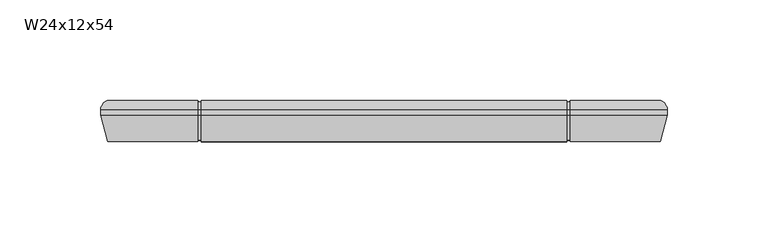
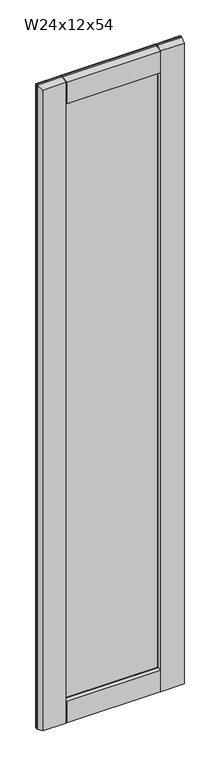
"""IFC4 building model written with IfcOpenShell, lengths in millimetres: furniture geometry, Cabinet-Wall-Merillat-Double_Door-Marlin : W24x12x54."""

from ifc_helpers import new_model, si_unit, frame, origin, place, context, project, spatial, polyline, circle_curve, ellipse_curve, outline, extrude, source, transform, mapped, element, save
from ifc_brep_helpers import plane_surface, cylinder_surface, advanced_brep


def w24x12x54_cfe01b16(model_context):
    return source(origin(), model_context, "Body", "SolidModel", [
        advanced_brep(
        [(541.0528392, 382.5621, 2108.2), (541.0528392, 382.5621, 787.4), (537.9563467, 387.0325, 790.4964925), (537.9563467, 387.0325, 2105.1035075), (541.0528392, 379.7935, 2108.2), (541.0528392, 379.7935, 787.4), (537.5476392, 366.7125, 2104.6948), (537.5476392, 366.7125, 790.9052), (492.8516765, 366.7125, 2059.9988372), (492.4815448, 367.50625, 2059.6287055), (490.4003857, 371.96931, 2057.5475465), (490.4003857, 371.96931, 838.0524535), (492.4815448, 367.50625, 835.9712945), (492.8516765, 366.7125, 835.6011628), (491.8001552, 374.2094093, 2058.947316), (491.8001552, 374.2094093, 836.652684), (506.1278392, 374.4595, 2073.275), (506.1278392, 374.4595, 822.325), (506.1278392, 379.2855, 2073.275), (506.1278392, 379.2855, 822.325), (491.8001552, 379.5355907, 2058.947316), (491.8001552, 379.5355907, 836.652684), (490.4003857, 381.77569, 2057.5475465), (490.4003857, 381.77569, 838.0524535), (492.4815448, 386.23875, 2059.6287055), (492.848809, 387.0263508, 2059.9959698), (492.8516765, 387.0325, 835.6011628), (492.4815448, 386.23875, 835.9712945), (263.1618317, 387.0325, 790.4964925), (308.2295579, 387.0325, 790.4964925), (308.2295579, 382.5621, 787.4), (260.0653392, 382.5621, 787.4), (492.848809, 382.5621, 787.4), (492.848809, 387.0325, 790.4964925), (491.261309, 382.5621, 787.4), (309.8170579, 382.5621, 787.4), (309.8170579, 387.0325, 790.4964925), (491.261309, 387.0325, 790.4964925), (308.2295579, 379.7935, 787.4), (260.0653392, 379.7935, 787.4), (492.848809, 379.7935, 787.4), (491.261309, 379.7935, 787.4), (309.8170579, 379.7935, 787.4), (308.2295579, 366.7125, 790.9052), (263.5705392, 366.7125, 790.9052), (491.261309, 366.7125, 790.9052), (309.8170579, 366.7125, 790.9052), (492.848809, 366.7125, 790.9052), (310.7177927, 371.96931, 838.0524535), (308.6366337, 367.50625, 835.9712945), (309.8170579, 367.50625, 835.9712945), (309.8170579, 366.7125, 835.6011628), (491.261309, 366.7125, 835.6011628), (491.261309, 367.50625, 835.9712945), (309.3180233, 374.2094093, 836.652684), (294.9903392, 374.4595, 822.325), (294.9903392, 379.2855, 822.325), (309.3180233, 379.5355907, 836.652684), (310.7177927, 381.77569, 838.0524535), (491.261309, 386.23875, 835.9712945), (491.261309, 387.0325, 835.6011628), (309.8170579, 387.0325, 835.6011628), (309.8170579, 386.23875, 835.9712945), (308.6366337, 386.23875, 835.9712945), (260.0653392, 382.5621, 2108.2), (263.1618317, 387.0325, 2105.1035075), (260.0653392, 379.7935, 2108.2), (263.5705392, 366.7125, 2104.6948), (308.266502, 366.7125, 835.6011628), (310.7177927, 371.96931, 2057.5475465), (308.6366337, 367.50625, 2059.6287055), (308.266502, 366.7125, 2059.9988372), (309.3180233, 374.2094093, 2058.947316), (294.9903392, 374.4595, 2073.275), (294.9903392, 379.2855, 2073.275), (309.3180233, 379.5355907, 2058.947316), (310.7177927, 381.77569, 2057.5475465), (308.266502, 387.0325, 835.6011628), (308.266502, 387.0325, 2059.9988372), (308.6366337, 386.23875, 2059.6287055), (492.848809, 387.0325, 2105.1035075), (492.848809, 382.5621, 2108.2), (308.2295579, 382.5621, 2108.2), (308.2295579, 387.0325, 2105.1035075), (309.8170579, 382.5621, 2108.2), (491.261309, 382.5621, 2108.2), (491.261309, 387.0325, 2105.1035075), (309.8170579, 387.0325, 2105.1035075), (492.848809, 379.7935, 2108.2), (308.2295579, 379.7935, 2108.2), (309.8170579, 379.7935, 2108.2), (491.261309, 379.7935, 2108.2), (492.848809, 366.7125, 2104.6948), (308.2295579, 366.7125, 2104.6948), (309.8170579, 366.7125, 2104.6948), (491.261309, 366.7125, 2104.6948), (309.8170579, 366.7125, 2059.9988372), (491.261309, 366.7125, 2059.9988372), (491.261309, 367.50625, 2059.6287055), (309.8170579, 367.50625, 2059.6287055), (309.8170579, 386.23875, 2059.6287055), (309.8170579, 387.0325, 2059.9988372), (491.261309, 387.0325, 2059.9988372), (491.261309, 386.23875, 2059.6287055), (309.8170579, 386.23875, 2104.9526052), (309.8170579, 382.5621, 2107.40625), (309.8170579, 379.8980037, 2107.40625), (309.8170579, 367.50625, 2104.0857412), (308.2295579, 367.50625, 2059.6287055), (308.2295579, 367.50625, 2104.0857412), (308.2295579, 379.8980037, 2107.40625), (308.2295579, 382.5621, 2107.40625), (308.2295579, 386.23875, 2104.9526052), (308.2295579, 386.23875, 2059.6287055), (492.848809, 386.23875, 2059.6287055), (492.848809, 386.23875, 2104.9526052), (492.848809, 382.5621, 2107.40625), (492.848809, 379.8980037, 2107.40625), (492.848809, 367.50625, 2104.0857412), (492.848809, 367.50625, 2059.6287055), (491.261309, 367.50625, 2104.0857412), (491.261309, 379.8980037, 2107.40625), (491.261309, 382.5621, 2107.40625), (491.261309, 386.23875, 2104.9526052), (492.848809, 367.50625, 835.9712945), (492.848809, 367.50625, 791.5142588), (492.848809, 379.8980037, 788.19375), (492.848809, 382.5621, 788.19375), (492.848809, 386.23875, 790.6473948), (492.848809, 386.23875, 835.9712945), (491.261309, 386.23875, 790.6473948), (491.261309, 382.5621, 788.19375), (491.261309, 379.8980037, 788.19375), (491.261309, 367.50625, 791.5142588), (309.8170579, 367.50625, 791.5142588), (309.8170579, 379.8980037, 788.19375), (309.8170579, 382.5621, 788.19375), (309.8170579, 386.23875, 790.6473948), (308.2295579, 386.23875, 835.9712945), (308.2295579, 386.23875, 790.6473948), (308.2295579, 382.5621, 788.19375), (308.2295579, 379.8980037, 788.19375), (308.2295579, 367.50625, 791.5142588), (308.2295579, 367.50625, 835.9712945)],
        [
            (0, 1),
            (1, 2, ellipse_curve(frame((536.2776392, 382.5621, 792.1752), z_axis=(0.7071067811865475, 0.0, 0.7071067811865475), x_axis=(-0.7071067811865474, 0.0, 0.7071067811865476)), 6.7531526, 4.7752)),
            (2, 3),
            (3, 0, ellipse_curve(frame((536.2776392, 382.5621, 2103.4248), z_axis=(0.7071067811865475, 0.0, -0.7071067811865475), x_axis=(0.7071067811865474, 0.0, 0.7071067811865476)), 6.7531526, 4.7752)),
            (0, 4),
            (4, 5),
            (5, 1),
            (4, 6),
            (6, 7),
            (7, 5),
            (8, 9),
            (9, 10),
            (10, 11),
            (11, 12),
            (12, 13),
            (13, 8),
            (10, 14, ellipse_curve(frame((491.8276392, 372.6348492, 2058.9748), z_axis=(0.7071067811865475, 0.0, -0.7071067811865475), x_axis=(0.7071067811865474, 0.0, 0.7071067811865476)), 2.2271035, 1.5748)),
            (14, 15),
            (15, 11, ellipse_curve(frame((491.8276392, 372.6348492, 836.6252), z_axis=(0.7071067811865475, 0.0, 0.7071067811865475), x_axis=(-0.7071067811865474, 0.0, 0.7071067811865476)), 2.2271035, 1.5748)),
            (14, 16),
            (16, 17),
            (17, 15),
            (16, 18),
            (18, 19),
            (19, 17),
            (18, 20),
            (20, 21),
            (21, 19),
            (20, 22, ellipse_curve(frame((491.8276392, 381.1101508, 2058.9748), z_axis=(0.7071067811865475, 0.0, -0.7071067811865475), x_axis=(0.7071067811865474, 0.0, 0.7071067811865476)), 2.2271035, 1.5748)),
            (22, 23),
            (23, 21, ellipse_curve(frame((491.8276392, 381.1101508, 836.6252), z_axis=(0.7071067811865475, 0.0, 0.7071067811865475), x_axis=(-0.7071067811865474, 0.0, 0.7071067811865476)), 2.2271035, 1.5748)),
            (22, 24),
            (24, 25),
            (25, 26),
            (26, 27),
            (27, 23),
            (28, 29),
            (29, 30, circle_curve(frame((308.2295579, 382.5621, 792.1752), z_axis=(-1.0, 0.0, 0.0), x_axis=(0.0, -1.0, 0.0)), 4.7752)),
            (30, 31),
            (31, 28, ellipse_curve(frame((264.8405392, 382.5621, 792.1752), z_axis=(0.7071067811865475, 0.0, -0.7071067811865475), x_axis=(0.7071067811865476, 0.0, 0.7071067811865474)), 6.7531526, 4.7752)),
            (1, 32),
            (32, 33, circle_curve(frame((492.848809, 382.5621, 792.1752), z_axis=(1.0, 0.0, 0.0), x_axis=(0.0, -1.0, 0.0)), 4.7752)),
            (33, 2),
            (34, 35),
            (35, 36, circle_curve(frame((309.8170579, 382.5621, 792.1752), z_axis=(1.0, 0.0, 0.0), x_axis=(0.0, -1.0, 0.0)), 4.7752)),
            (36, 37),
            (37, 34, circle_curve(frame((491.261309, 382.5621, 792.1752), z_axis=(-1.0, 0.0, 0.0), x_axis=(0.0, -1.0, 0.0)), 4.7752)),
            (30, 38),
            (38, 39),
            (39, 31),
            (5, 40),
            (40, 32),
            (41, 42),
            (42, 35),
            (34, 41),
            (38, 43),
            (43, 44),
            (44, 39),
            (45, 46),
            (46, 42),
            (41, 45),
            (7, 47),
            (47, 40),
            (48, 49),
            (49, 50),
            (50, 51),
            (51, 52),
            (52, 53),
            (53, 12),
            (11, 48),
            (15, 54),
            (54, 48, ellipse_curve(frame((309.2905392, 372.6348492, 836.6252), z_axis=(0.7071067811865475, 0.0, -0.7071067811865475), x_axis=(0.7071067811865476, 0.0, 0.7071067811865474)), 2.2271035, 1.5748)),
            (17, 55),
            (55, 54),
            (19, 56),
            (56, 55),
            (21, 57),
            (57, 56),
            (23, 58),
            (58, 57, ellipse_curve(frame((309.2905392, 381.1101508, 836.6252), z_axis=(0.7071067811865475, 0.0, -0.7071067811865475), x_axis=(0.7071067811865476, 0.0, 0.7071067811865474)), 2.2271035, 1.5748)),
            (27, 59),
            (59, 60),
            (60, 61),
            (61, 62),
            (62, 63),
            (63, 58),
            (31, 64),
            (64, 65, ellipse_curve(frame((264.8405392, 382.5621, 2103.4248), z_axis=(-0.7071067811865475, 0.0, -0.7071067811865475), x_axis=(0.7071067811865474, 0.0, -0.7071067811865476)), 6.7531526, 4.7752)),
            (65, 28),
            (39, 66),
            (66, 64),
            (44, 67),
            (67, 66),
            (68, 49),
            (48, 69),
            (69, 70),
            (70, 71),
            (71, 68),
            (54, 72),
            (72, 69, ellipse_curve(frame((309.2905392, 372.6348492, 2058.9748), z_axis=(-0.7071067811865475, 0.0, -0.7071067811865475), x_axis=(0.7071067811865474, 0.0, -0.7071067811865476)), 2.2271035, 1.5748)),
            (55, 73),
            (73, 72),
            (56, 74),
            (74, 73),
            (57, 75),
            (75, 74),
            (58, 76),
            (76, 75, ellipse_curve(frame((309.2905392, 381.1101508, 2058.9748), z_axis=(-0.7071067811865475, 0.0, -0.7071067811865475), x_axis=(0.7071067811865474, 0.0, -0.7071067811865476)), 2.2271035, 1.5748)),
            (63, 77),
            (77, 78),
            (78, 79),
            (79, 76),
            (3, 80),
            (80, 81, circle_curve(frame((492.848809, 382.5621, 2103.4248), z_axis=(1.0, 0.0, 0.0), x_axis=(0.0, -1.0, 0.0)), 4.7752)),
            (81, 0),
            (64, 82),
            (82, 83, circle_curve(frame((308.2295579, 382.5621, 2103.4248), z_axis=(-1.0, 0.0, 0.0), x_axis=(0.0, -1.0, 0.0)), 4.7752)),
            (83, 65),
            (84, 85),
            (85, 86, circle_curve(frame((491.261309, 382.5621, 2103.4248), z_axis=(-1.0, 0.0, 0.0), x_axis=(0.0, -1.0, 0.0)), 4.7752)),
            (86, 87),
            (87, 84, circle_curve(frame((309.8170579, 382.5621, 2103.4248), z_axis=(1.0, 0.0, 0.0), x_axis=(0.0, -1.0, 0.0)), 4.7752)),
            (81, 88),
            (88, 4),
            (66, 89),
            (89, 82),
            (90, 91),
            (91, 85),
            (84, 90),
            (88, 92),
            (92, 6),
            (67, 93),
            (93, 89),
            (94, 95),
            (95, 91),
            (90, 94),
            (51, 46),
            (45, 52),
            (43, 68),
            (71, 93),
            (92, 8),
            (13, 47),
            (96, 97),
            (97, 95),
            (94, 96),
            (9, 98),
            (98, 97),
            (96, 99),
            (99, 70),
            (69, 10),
            (72, 14),
            (73, 16),
            (74, 18),
            (75, 20),
            (76, 22),
            (79, 100),
            (100, 101),
            (101, 102),
            (102, 103),
            (103, 24),
            (33, 26),
            (25, 80),
            (36, 61),
            (60, 37),
            (83, 78),
            (77, 29),
            (86, 102),
            (101, 87),
            (100, 104),
            (104, 105, circle_curve(frame((309.8170579, 382.5621, 2103.4248), z_axis=(1.0, 0.0, 0.0), x_axis=(0.0, 0.0, 1.0)), 3.98145)),
            (105, 106),
            (106, 107),
            (107, 99),
            (71, 108),
            (108, 109),
            (109, 110),
            (110, 111),
            (111, 112, circle_curve(frame((308.2295579, 382.5621, 2103.4248), z_axis=(-1.0, 0.0, 0.0), x_axis=(0.0, 0.0, 1.0)), 3.98145)),
            (112, 113),
            (113, 78),
            (113, 79),
            (112, 104),
            (111, 105),
            (110, 106),
            (109, 107),
            (108, 70),
            (25, 114),
            (114, 115),
            (115, 116, circle_curve(frame((492.848809, 382.5621, 2103.4248), z_axis=(1.0, 0.0, 0.0), x_axis=(0.0, 0.0, 1.0)), 3.98145)),
            (116, 117),
            (117, 118),
            (118, 119),
            (119, 8),
            (98, 120),
            (120, 121),
            (121, 122),
            (122, 123, circle_curve(frame((491.261309, 382.5621, 2103.4248), z_axis=(-1.0, 0.0, 0.0), x_axis=(0.0, 0.0, 1.0)), 3.98145)),
            (123, 103),
            (24, 114),
            (123, 115),
            (122, 116),
            (121, 117),
            (120, 118),
            (9, 119),
            (13, 124),
            (124, 125),
            (125, 126),
            (126, 127),
            (127, 128, circle_curve(frame((492.848809, 382.5621, 792.1752), z_axis=(1.0, 0.0, 0.0), x_axis=(0.0, 0.0, 1.0)), 3.98145)),
            (128, 129),
            (129, 26),
            (59, 130),
            (130, 131, circle_curve(frame((491.261309, 382.5621, 792.1752), z_axis=(-1.0, 0.0, 0.0), x_axis=(0.0, 0.0, 1.0)), 3.98145)),
            (131, 132),
            (132, 133),
            (133, 53),
            (12, 124),
            (133, 125),
            (132, 126),
            (131, 127),
            (130, 128),
            (27, 129),
            (50, 134),
            (134, 135),
            (135, 136),
            (136, 137, circle_curve(frame((309.8170579, 382.5621, 792.1752), z_axis=(1.0, 0.0, 0.0), x_axis=(0.0, 0.0, 1.0)), 3.98145)),
            (137, 62),
            (138, 139),
            (139, 140, circle_curve(frame((308.2295579, 382.5621, 792.1752), z_axis=(-1.0, 0.0, 0.0), x_axis=(0.0, 0.0, 1.0)), 3.98145)),
            (140, 141),
            (141, 142),
            (142, 143),
            (143, 68),
            (77, 138),
            (63, 138),
            (143, 49),
            (142, 134),
            (141, 135),
            (140, 136),
            (139, 137),
        ],
        [
            cylinder_surface(frame((536.2776392, 382.5621, 2108.2), z_axis=(0.0, 0.0, 1.0), x_axis=(0.0, -1.0, 0.0)), 4.7752),
            plane_surface(frame((541.0528392, 382.5621, 2108.2), z_axis=(1.0, 0.0, 0.0), x_axis=(0.0, 0.0, -1.0))),
            plane_surface(frame((541.0528392, 379.7935, 2108.2), z_axis=(0.9659229350723619, -0.25882983502910506, 0.0), x_axis=(0.0, 0.0, -1.0))),
            plane_surface(frame((492.8516765, 366.7125, 2059.9988372), z_axis=(-0.9063077870366099, -0.4226182617407856, 0.0), x_axis=(0.0, 0.0, -1.0))),
            cylinder_surface(frame((491.8276392, 372.6348492, 2108.2), z_axis=(0.0, 0.0, 1.0000000000000002), x_axis=(-0.01745240643729364, 0.9998476951563912, 0.0)), 1.5748),
            plane_surface(frame((491.8001552, 374.2094093, 2058.947316), z_axis=(-0.017452406437322144, 0.9998476951563906, 0.0), x_axis=(0.0, 0.0, -1.0))),
            plane_surface(frame((506.1278392, 374.4595, 2073.275), z_axis=(-1.0, 0.0, 0.0), x_axis=(0.0, 0.0, -1.0))),
            plane_surface(frame((506.1278392, 379.2855, 2073.275), z_axis=(-0.01745240643727848, -0.9998476951563914, 0.0), x_axis=(0.0, 0.0, -1.0))),
            cylinder_surface(frame((491.8276392, 381.1101508, 2108.2), z_axis=(0.0, 0.0, 1.0000000000000002), x_axis=(-0.9063077870367326, 0.42261826174052236, 0.0)), 1.5748),
            plane_surface(frame((490.4003857, 381.77569, 2057.5475465), z_axis=(-0.9063077870366333, 0.4226182617407352, 0.0), x_axis=(0.0, 0.0, -1.0))),
            cylinder_surface(frame((541.0528392, 382.5621, 792.1752), z_axis=(1.0, 0.0, 0.0), x_axis=(0.0, -1.0, 0.0)), 4.7752),
            plane_surface(frame((541.0528392, 382.5621, 787.4), z_axis=(0.0, 0.0, -1.0), x_axis=(-1.0, 0.0, 0.0))),
            plane_surface(frame((541.0528392, 379.7935, 787.4), z_axis=(0.0, -0.2588298350291095, -0.9659229350723607), x_axis=(-1.0, 0.0, 0.0))),
            plane_surface(frame((492.8516765, 366.7125, 835.6011628), z_axis=(0.0, -0.42261826174078143, 0.9063077870366119), x_axis=(-1.0, 0.0, 0.0))),
            cylinder_surface(frame((541.0528392, 372.6348492, 836.6252), z_axis=(1.0000000000000002, 0.0, 0.0), x_axis=(0.0, 0.9998476951563913, 0.017452406437289025)), 1.5748),
            plane_surface(frame((491.8001552, 374.2094093, 836.652684), z_axis=(0.0, 0.9998476951563907, 0.01745240643731753), x_axis=(-1.0, 0.0, 0.0))),
            plane_surface(frame((506.1278392, 374.4595, 822.325), z_axis=(0.0, 0.0, 1.0), x_axis=(-1.0, 0.0, 0.0))),
            plane_surface(frame((506.1278392, 379.2855, 822.325), z_axis=(0.0, -0.9998476951563913, 0.017452406437283095), x_axis=(-1.0, 0.0, 0.0))),
            cylinder_surface(frame((541.0528392, 381.1101508, 836.6252), z_axis=(1.0000000000000002, 0.0, 0.0), x_axis=(0.0, 0.4226182617405265, 0.9063077870367306)), 1.5748),
            plane_surface(frame((490.4003857, 381.77569, 838.0524535), z_axis=(0.0, 0.4226182617407394, 0.9063077870366314), x_axis=(-1.0, 0.0, 0.0))),
            cylinder_surface(frame((264.8405392, 382.5621, 787.4), z_axis=(0.0, 0.0, -1.0), x_axis=(0.0, -1.0, 0.0)), 4.7752),
            plane_surface(frame((260.0653392, 382.5621, 787.4), z_axis=(-1.0, 0.0, 0.0), x_axis=(0.0, 0.0, 1.0))),
            plane_surface(frame((260.0653392, 379.7935, 787.4), z_axis=(-0.9659229350723619, -0.25882983502910506, 0.0), x_axis=(0.0, 0.0, 1.0))),
            plane_surface(frame((308.266502, 366.7125, 835.6011628), z_axis=(0.9063077870366099, -0.4226182617407856, 0.0), x_axis=(0.0, 0.0, 1.0))),
            cylinder_surface(frame((309.2905392, 372.6348492, 787.4), z_axis=(0.0, 0.0, -1.0000000000000002), x_axis=(0.01745240643729364, 0.9998476951563912, 0.0)), 1.5748),
            plane_surface(frame((309.3180233, 374.2094093, 836.652684), z_axis=(0.017452406437322144, 0.9998476951563906, 0.0), x_axis=(0.0, 0.0, 1.0))),
            plane_surface(frame((294.9903392, 374.4595, 822.325), z_axis=(1.0, 0.0, 0.0), x_axis=(0.0, 0.0, 1.0))),
            plane_surface(frame((294.9903392, 379.2855, 822.325), z_axis=(0.01745240643727848, -0.9998476951563914, 0.0), x_axis=(0.0, 0.0, 1.0))),
            cylinder_surface(frame((309.2905392, 381.1101508, 787.4), z_axis=(0.0, 0.0, -1.0000000000000002), x_axis=(0.9063077870367326, 0.42261826174052236, 0.0)), 1.5748),
            plane_surface(frame((310.7177927, 381.77569, 838.0524535), z_axis=(0.9063077870366333, 0.4226182617407352, 0.0), x_axis=(0.0, 0.0, 1.0))),
            cylinder_surface(frame((260.0653392, 382.5621, 2103.4248), z_axis=(-1.0, 0.0, 0.0), x_axis=(0.0, -1.0, 0.0)), 4.7752),
            plane_surface(frame((260.0653392, 382.5621, 2108.2), z_axis=(0.0, 0.0, 1.0), x_axis=(1.0, 0.0, 0.0))),
            plane_surface(frame((260.0653392, 379.7935, 2108.2), z_axis=(0.0, -0.2588298350291006, 0.9659229350723632), x_axis=(1.0, 0.0, 0.0))),
            plane_surface(frame((263.5705392, 366.7125, 2104.6948), z_axis=(0.0, -1.0, 0.0), x_axis=(1.0, 0.0, 0.0))),
            plane_surface(frame((308.266502, 366.7125, 2059.9988372), z_axis=(0.0, -0.42261826174078976, -0.9063077870366079), x_axis=(1.0, 0.0, 0.0))),
            cylinder_surface(frame((260.0653392, 372.6348492, 2058.9748), z_axis=(-1.0000000000000002, 0.0, 0.0), x_axis=(0.0, 0.999847695156391, -0.017452406437298253)), 1.5748),
            plane_surface(frame((309.3180233, 374.2094093, 2058.947316), z_axis=(0.0, 0.9998476951563905, -0.01745240643732676), x_axis=(1.0, 0.0, 0.0))),
            plane_surface(frame((294.9903392, 374.4595, 2073.275), z_axis=(0.0, 0.0, -1.0), x_axis=(1.0, 0.0, 0.0))),
            plane_surface(frame((294.9903392, 379.2855, 2073.275), z_axis=(0.0, -0.9998476951563915, -0.017452406437273867), x_axis=(1.0, 0.0, 0.0))),
            cylinder_surface(frame((260.0653392, 381.1101508, 2058.9748), z_axis=(-1.0000000000000002, 0.0, 0.0), x_axis=(0.0, 0.4226182617405182, -0.9063077870367346)), 1.5748),
            plane_surface(frame((310.7177927, 381.77569, 2057.5475465), z_axis=(0.0, 0.422618261740731, -0.9063077870366353), x_axis=(1.0, 0.0, 0.0))),
            plane_surface(frame((308.266502, 387.0325, 2059.9988372), z_axis=(0.0, 1.0, 0.0), x_axis=(1.0, 0.0, 0.0))),
            plane_surface(frame((309.8170579, 387.0325, 2059.9988372), z_axis=(-1.0000000000000002, 0.0, 0.0), x_axis=(0.0, -0.9063077870366177, -0.4226182617407689))),
            plane_surface(frame((308.2295579, 387.0325, 2059.9988372), z_axis=(1.0000000000000002, 0.0, 0.0), x_axis=(0.0, 0.9063077870366177, 0.4226182617407689))),
            plane_surface(frame((309.8170579, 387.0325, 2059.9988372), z_axis=(0.0, -0.4226182617407689, 0.9063077870366177), x_axis=(-1.0, 0.0, 0.0))),
            plane_surface(frame((309.8170579, 386.23875, 2059.6287055), z_axis=(0.0, 1.0, 0.0), x_axis=(-1.0, 0.0, 0.0))),
            cylinder_surface(frame((308.2295579, 382.5621, 2103.4248), z_axis=(-1.0, 0.0, 0.0), x_axis=(0.0, 0.0, 1.0)), 3.98145),
            plane_surface(frame((309.8170579, 382.5621, 2107.40625), z_axis=(0.0, 0.0, 1.0), x_axis=(-1.0, 0.0, 0.0))),
            plane_surface(frame((309.8170579, 379.8980037, 2107.40625), z_axis=(0.0, -0.2588298350291571, 0.965922935072348), x_axis=(-1.0, 0.0, 0.0))),
            plane_surface(frame((309.8170579, 367.50625, 2104.0857412), z_axis=(0.0, -1.0, 0.0), x_axis=(-1.0, 0.0, 0.0))),
            plane_surface(frame((309.8170579, 367.50625, 2059.6287055), z_axis=(0.0, 0.4226182617408151, 0.906307787036596), x_axis=(-1.0, 0.0, 0.0))),
            plane_surface(frame((492.848809, 387.0325, 2059.9988372), z_axis=(-1.0, 0.0, 0.0), x_axis=(0.0, -0.9063077870366254, -0.42261826174075223))),
            plane_surface(frame((491.261309, 387.0325, 2059.9988372), z_axis=(1.0, 0.0, 0.0), x_axis=(0.0, 0.9063077870366254, 0.42261826174075223))),
            plane_surface(frame((492.848809, 387.0325, 2059.9988372), z_axis=(0.0, -0.42261826174075223, 0.9063077870366254), x_axis=(-1.0, 0.0, 0.0))),
            plane_surface(frame((492.848809, 386.23875, 2059.6287055), z_axis=(0.0, 1.0, 0.0), x_axis=(-1.0, 0.0, 0.0))),
            cylinder_surface(frame((491.261309, 382.5621, 2103.4248), z_axis=(-1.0, 0.0, 0.0), x_axis=(0.0, 0.0, 1.0)), 3.98145),
            plane_surface(frame((492.848809, 382.5621, 2107.40625), z_axis=(0.0, 0.0, 1.0), x_axis=(-1.0, 0.0, 0.0))),
            plane_surface(frame((492.848809, 379.8980037, 2107.40625), z_axis=(0.0, -0.258829835029159, 0.9659229350723475), x_axis=(-1.0, 0.0, 0.0))),
            plane_surface(frame((492.848809, 367.50625, 2104.0857412), z_axis=(0.0, -1.0, 0.0), x_axis=(-1.0, 0.0, 0.0))),
            plane_surface(frame((492.848809, 367.50625, 2059.6287055), z_axis=(0.0, 0.4226182617408322, 0.9063077870365881), x_axis=(-1.0, 0.0, 0.0))),
            plane_surface(frame((492.848809, 382.5621, 796.9504), z_axis=(-1.0, 0.0, 0.0), x_axis=(0.0, 1.0, 0.0))),
            plane_surface(frame((491.261309, 382.5621, 796.9504), z_axis=(1.0, 0.0, 0.0), x_axis=(0.0, -1.0, 0.0))),
            plane_surface(frame((492.848809, 366.7125, 835.6011628), z_axis=(0.0, 0.4226182617407559, -0.9063077870366237), x_axis=(-1.0, 0.0, 0.0))),
            plane_surface(frame((492.848809, 367.50625, 835.9712945), z_axis=(0.0, -1.0, 0.0), x_axis=(-1.0, 0.0, 0.0))),
            plane_surface(frame((492.848809, 367.50625, 791.5142588), z_axis=(0.0, -0.25882983502944146, -0.9659229350722718), x_axis=(-1.0, 0.0, 0.0))),
            plane_surface(frame((492.848809, 379.8980037, 788.19375), z_axis=(0.0, 0.0, -1.0), x_axis=(-1.0, 0.0, 0.0))),
            cylinder_surface(frame((491.261309, 382.5621, 792.1752), z_axis=(-1.0, 0.0, 0.0), x_axis=(0.0, 0.0, 1.0)), 3.98145),
            plane_surface(frame((492.848809, 386.23875, 790.6473948), z_axis=(0.0, 1.0, 0.0), x_axis=(-1.0, 0.0, 0.0))),
            plane_surface(frame((492.848809, 386.23875, 835.9712945), z_axis=(0.0, -0.42261826174073325, -0.9063077870366342), x_axis=(-1.0, 0.0, 0.0))),
            plane_surface(frame((309.8170579, 386.23875, 835.9712945), z_axis=(-1.0, 0.0, 0.0), x_axis=(0.0, 0.9063077870366539, -0.42261826174069095))),
            plane_surface(frame((308.2295579, 386.23875, 835.9712945), z_axis=(1.0, 0.0, 0.0), x_axis=(0.0, -0.9063077870366539, 0.42261826174069095))),
            plane_surface(frame((309.8170579, 386.23875, 835.9712945), z_axis=(0.0, -0.42261826174069095, -0.9063077870366539), x_axis=(-1.0, 0.0, 0.0))),
            plane_surface(frame((309.8170579, 366.7125, 835.6011628), z_axis=(0.0, 0.42261826174079387, -0.9063077870366061), x_axis=(-1.0, 0.0, 0.0))),
            plane_surface(frame((309.8170579, 367.50625, 835.9712945), z_axis=(0.0, -1.0, 0.0), x_axis=(-1.0, 0.0, 0.0))),
            plane_surface(frame((309.8170579, 367.50625, 791.5142588), z_axis=(0.0, -0.25882983502944, -0.9659229350722722), x_axis=(-1.0, 0.0, 0.0))),
            plane_surface(frame((309.8170579, 379.8980037, 788.19375), z_axis=(0.0, 0.0, -1.0), x_axis=(-1.0, 0.0, 0.0))),
            cylinder_surface(frame((308.2295579, 382.5621, 792.1752), z_axis=(-1.0, 0.0, 0.0), x_axis=(0.0, 0.0, 1.0)), 3.98145),
            plane_surface(frame((309.8170579, 386.23875, 790.6473948), z_axis=(0.0, 1.0, 0.0), x_axis=(-1.0, 0.0, 0.0))),
        ],
        [
            (0, [[1, 2, 3, 4]]),
            (1, [[5, 6, 7, -1]]),
            (2, [[8, 9, 10, -6]]),
            (3, [[11, 12, 13, 14, 15, 16]]),
            (4, [[17, 18, 19, -13]]),
            (5, [[20, 21, 22, -18]]),
            (6, [[23, 24, 25, -21]]),
            (7, [[26, 27, 28, -24]]),
            (8, [[29, 30, 31, -27]]),
            (9, [[32, 33, 34, 35, 36, -30]]),
            (10, [[37, 38, 39, 40]]),
            (10, [[41, 42, 43, -2]]),
            (10, [[44, 45, 46, 47]]),
            (11, [[-39, 48, 49, 50]]),
            (11, [[51, 52, -41, -7]]),
            (11, [[53, 54, -44, 55]]),
            (12, [[-49, 56, 57, 58]]),
            (12, [[59, 60, -53, 61]]),
            (12, [[62, 63, -51, -10]]),
            (13, [[64, 65, 66, 67, 68, 69, -14, 70]]),
            (14, [[71, 72, -70, -19]]),
            (15, [[73, 74, -71, -22]]),
            (16, [[75, 76, -73, -25]]),
            (17, [[77, 78, -75, -28]]),
            (18, [[79, 80, -77, -31]]),
            (19, [[-36, 81, 82, 83, 84, 85, 86, -79]]),
            (20, [[87, 88, 89, -40]]),
            (21, [[90, 91, -87, -50]]),
            (22, [[92, 93, -90, -58]]),
            (23, [[94, -64, 95, 96, 97, 98]]),
            (24, [[99, 100, -95, -72]]),
            (25, [[101, 102, -99, -74]]),
            (26, [[103, 104, -101, -76]]),
            (27, [[105, 106, -103, -78]]),
            (28, [[107, 108, -105, -80]]),
            (29, [[-86, 109, 110, 111, 112, -107]]),
            (30, [[113, 114, 115, -4]]),
            (30, [[116, 117, 118, -88]]),
            (30, [[119, 120, 121, 122]]),
            (31, [[-115, 123, 124, -5]]),
            (31, [[125, 126, -116, -91]]),
            (31, [[127, 128, -119, 129]]),
            (32, [[-124, 130, 131, -8]]),
            (32, [[132, 133, -125, -93]]),
            (32, [[134, 135, -127, 136]]),
            (33, [[-67, 137, -59, 138]]),
            (33, [[-57, 139, -98, 140, -132, -92]]),
            (33, [[-131, 141, -16, 142, -62, -9]]),
            (33, [[143, 144, -134, 145]]),
            (34, [[-12, 146, 147, -143, 148, 149, -96, 150]]),
            (35, [[-150, -100, 151, -17]]),
            (36, [[-151, -102, 152, -20]]),
            (37, [[-152, -104, 153, -23]]),
            (38, [[-153, -106, 154, -26]]),
            (39, [[-154, -108, 155, -29]]),
            (40, [[-112, 156, 157, 158, 159, 160, -32, -155]]),
            (41, [[-43, 161, -34, 162, -113, -3]]),
            (41, [[-46, 163, -83, 164]]),
            (41, [[-118, 165, -110, 166, -37, -89]]),
            (41, [[-121, 167, -158, 168]]),
            (42, [[-148, -145, -136, -129, -122, -168, -157, 169, 170, 171, 172, 173]]),
            (43, [[-165, -117, -126, -133, -140, 174, 175, 176, 177, 178, 179, 180]]),
            (44, [[181, -111, -180]]),
            (45, [[-156, -181, -179, 182, -169]]),
            (46, [[-182, -178, 183, -170]]),
            (47, [[-183, -177, 184, -171]]),
            (48, [[-184, -176, 185, -172]]),
            (49, [[-185, -175, 186, -149, -173]]),
            (50, [[-97, -186, -174]]),
            (51, [[-141, -130, -123, -114, -162, 187, 188, 189, 190, 191, 192, 193]]),
            (52, [[-159, -167, -120, -128, -135, -144, -147, 194, 195, 196, 197, 198]]),
            (53, [[-33, 199, -187]]),
            (54, [[-199, -160, -198, 200, -188]]),
            (55, [[-200, -197, 201, -189]]),
            (56, [[-201, -196, 202, -190]]),
            (57, [[-202, -195, 203, -191]]),
            (58, [[-203, -194, -146, 204, -192]]),
            (59, [[-204, -11, -193]]),
            (60, [[-161, -42, -52, -63, -142, 205, 206, 207, 208, 209, 210, 211]]),
            (61, [[-68, -138, -61, -55, -47, -164, -82, 212, 213, 214, 215, 216]]),
            (62, [[-15, 217, -205]]),
            (63, [[-217, -69, -216, 218, -206]]),
            (64, [[-218, -215, 219, -207]]),
            (65, [[-219, -214, 220, -208]]),
            (66, [[-220, -213, 221, -209]]),
            (67, [[-221, -212, -81, 222, -210]]),
            (68, [[-222, -35, -211]]),
            (69, [[-84, -163, -45, -54, -60, -137, -66, 223, 224, 225, 226, 227]]),
            (70, [[228, 229, 230, 231, 232, 233, -139, -56, -48, -38, -166, 234]]),
            (71, [[-109, 235, -234]]),
            (72, [[236, -94, -233]]),
            (73, [[-65, -236, -232, 237, -223]]),
            (74, [[-237, -231, 238, -224]]),
            (75, [[-238, -230, 239, -225]]),
            (76, [[-239, -229, 240, -226]]),
            (77, [[-240, -228, -235, -85, -227]]),
        ],
    ),
        extrude(outline(polyline([(294.9903392, 379.2855), (506.1278392, 379.2855), (506.1278392, 374.4595), (294.9903392, 374.4595), (294.9903392, 379.2855)])), frame((0.0, 0.0, 822.325), z_axis=(0.0, 0.0, 1.0), x_axis=(1.0, 0.0, 0.0)), (0.0, 0.0, 1.0), 1250.95),
    ])


if __name__ == "__main__":
    model = new_model("IFC4")
    model_context = context("Model", 3, world=origin())
    ifc_project = project(units=[si_unit("LENGTHUNIT", "METRE", prefix="MILLI")], contexts=[model_context])
    site = spatial("IfcSite", under=ifc_project)
    building = spatial("IfcBuilding", under=site)
    placement = place(None, origin())
    w24x12x54_shape = w24x12x54_cfe01b16(model_context)
    element("IfcFurniture", 1, ObjectType="Cabinet-Wall-Merillat-Double_Door-Marlin : W24x12x54", at=placement, inside=building, context=model_context, shape_type="MappedRepresentation", body=[
        mapped(w24x12x54_shape, transform((0.0, 0.0, 0.0), x_axis=(1.0, 0.0, 0.0), y_axis=(0.0, 1.0, 0.0), z_axis=(0.0, 0.0, 1.0))),
    ])
    save(model, "model.ifc")

# Revit data of these elements
# Type "Cabinet-Wall-Merillat-Double_Door-Marlin : W24x12x54"
#   URL = "https://www.merillat.com/"
#   Product Page URL = "https://www.merillat.com/our-products/"
#   Product Line = "Express"
#   Product Group = "Wall Cabinet"
#   Product Documentation Link = "http://merillatbusiness.com/wp-content/uploads/2014/07/Merillat_Classic_Catalog.pdf"
#   Model = "W2442B"
#   Manufacturer = "Merillat"
#   Height Note = "Actual Height of 21 inches Cabinet is 20 1/2 inches"
#   Glass Door Note = "Glass Cabinet doors are only available in specific sizes. Please refer to the catalog for this information before requesting a glass size."
#   Finish = "Wood"
#   Description = "Wall 2442 Butt Door"
#   Construction Type = "Wall Cabinet"
#   Cabinet Construction Note = "Cabinets with B suffix have BUTT doors without a center frame stile:"
#   Assembly Code = "C1030410"
#   Spacing = 0' - 1"
#   Shelving Height = 1' - 0 3/4"
#   Door Spacing = 0' - 0 1/8"
#   Cabinet Door Width = 0' - 11 1/16"
#   Cabinet Door Height = 4' - 4"
#   Depth = 1' - 0"
#   Height = 4' - 6"
#   Top Of Cabinet = 7' - 0"
#   Width = 2' - 0"
#   COBie.Type = no
#   Top and Bottom Visibility = yes
#   Partial Overlay Butt = yes
#   Partial Overlay = no
#   Number of Shelves Greater than one = 3
#   Number of Shelves = 3
#   Middle Shelf = yes
#   Full Overlay Butt = no
#   Full Overlay = no
#   Elevation Swing Line = yes
#   Door Drawer Material = Wood - Merillat - Pecan(1)
#   Cabinet Material = Wood - Merillat - Pecan(1)
#   Cabinet Door Style = element 806847
# Element 1 (IfcFurniture, "Cabinet-Wall-Merillat-Double_Door-Marlin : W24x12x54")
#   Materials on its faces: "Wood - Merillat - Pecan(1)"
# Materials
#   "Wood - Merillat - Pecan(1)": class "Wood", colour RGB 108 67 43, transparency 0, Cost = 0
